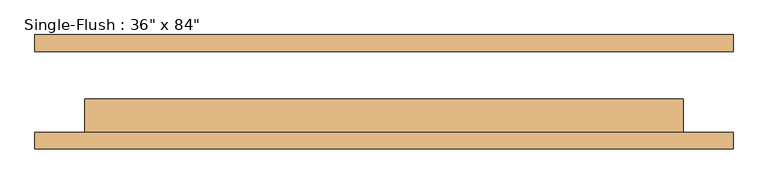
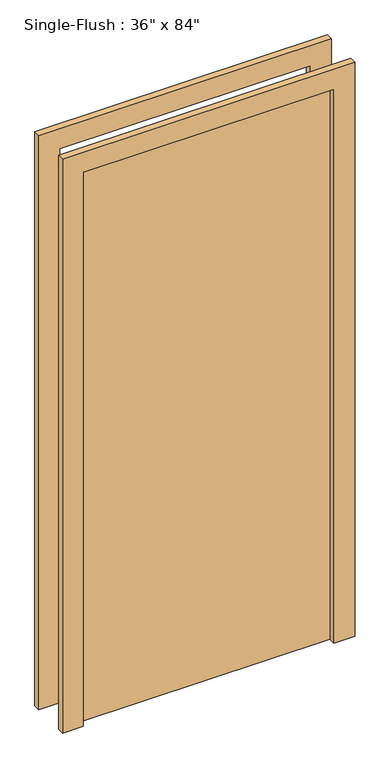
"""IFC4 building model written with IfcOpenShell, lengths in millimetres: door geometry."""

from ifc_helpers import new_model, si_unit, frame, origin, origin_with_axes, place, context, project, spatial, polyline, outline, extrude, source, transform, mapped, element, save


def door_eb9f8b14(model_context):
    return source(origin(), model_context, "Body", "SweptSolid", [
        extrude(outline(polyline([(2209.8, -533.4), (0.0, -533.4), (0.0, -457.2), (2133.6, -457.2), (2133.6, 457.2), (0.0, 457.2), (0.0, 533.4), (2209.8, 533.4), (2209.8, -533.4)])), frame((0.0, -87.3125, 0.0), z_axis=(0.0, 1.0, 0.0), x_axis=(0.0, 0.0, 1.0)), (0.0, 0.0, 1.0), 25.4),
        extrude(outline(polyline([(2209.8, 533.4), (2209.8, -533.4), (0.0, -533.4), (0.0, -457.2), (2133.6, -457.2), (2133.6, 457.2), (0.0, 457.2), (0.0, 533.4), (2209.8, 533.4)])), frame((0.0, 61.9125, 0.0), z_axis=(0.0, 1.0, 0.0), x_axis=(0.0, 0.0, 1.0)), (0.0, 0.0, 1.0), 25.4),
        extrude(outline(polyline([(457.2, -11.1125), (457.2, -61.9125), (-457.2, -61.9125), (-457.2, -11.1125), (457.2, -11.1125)])), origin_with_axes(), (0.0, 0.0, 1.0), 2133.6),
    ])


if __name__ == "__main__":
    model = new_model("IFC4")
    model_context = context("Model", 3, world=origin())
    ifc_project = project(units=[si_unit("LENGTHUNIT", "METRE", prefix="MILLI")], contexts=[model_context])
    site = spatial("IfcSite", under=ifc_project)
    building = spatial("IfcBuilding", under=site)
    placement = place(None, origin())
    door_shape = door_eb9f8b14(model_context)
    element("IfcDoor", 1, ObjectType="Single-Flush : 36\" x 84\"", at=placement, inside=building, context=model_context, shape_type="MappedRepresentation", body=[
        mapped(door_shape, transform((0.0, 0.0, 0.0), x_axis=(1.0, 0.0, 0.0), y_axis=(0.0, 1.0, 0.0), z_axis=(0.0, 0.0, 1.0))),
    ])
    save(model, "model.ifc")

# Revit data of these elements
# Type "Single-Flush : 36\" x 84\""
#   Type Mark = "1"
#   Assembly Code = "C1020"
#   Thickness = 0' - 2"
#   Height = 7' - 0"
#   Trim Projection Ext = 0' - 1"
#   Trim Projection Int = 0' - 1"
#   Trim Width = 0' - 3"
#   Width = 3' - 0"
#   Door Material = none
#   Frame Material = none
#   Function = (empty or 0)
#   Wall Closure = (empty or 0)
